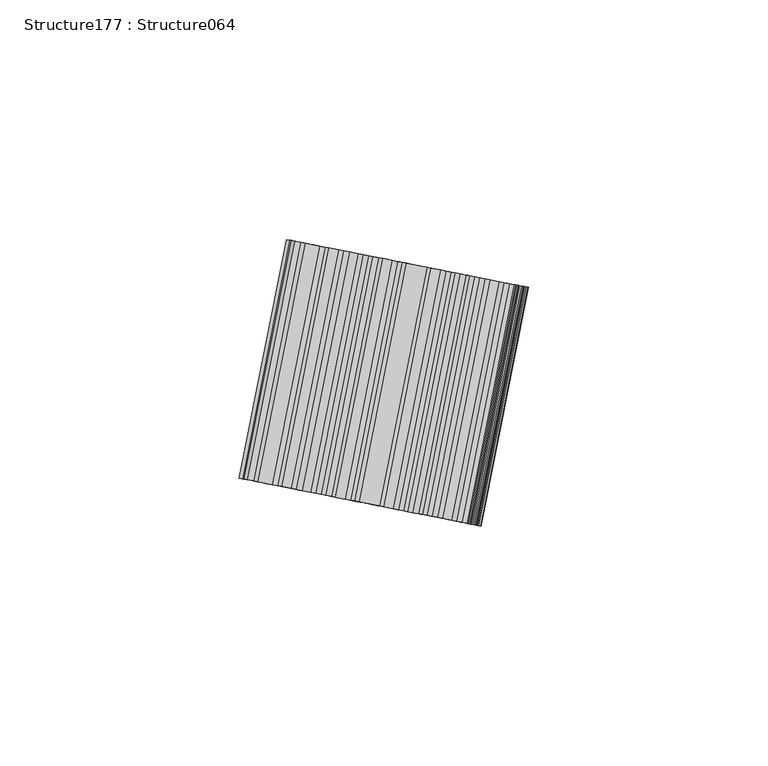
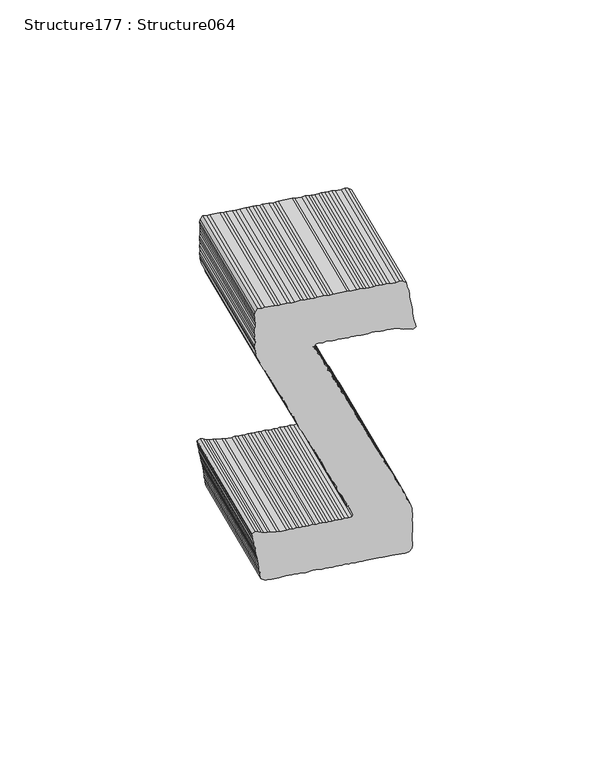
"""IFC4 building model written with IfcOpenShell, lengths in millimetres: proxy geometry, Structure177 : Structure064."""

from ifc_helpers import new_model, si_unit, frame, origin, place, context, project, spatial, polyline, outline, extrude, source, transform, mapped, element, save


def structure177_structure064_2659b349(model_context):
    return source(origin(), model_context, "Body", "SweptSolid", [
        extrude(outline(polyline([(1.0468911, 0.0), (1.5156229, -1.0820274), (1.8043049, -2.1128067), (2.0901183, -3.1435853), (2.6051551, -4.0455174), (2.8493861, -5.2553333), (3.1877265, -6.1090195), (3.6541636, -7.1898987), (3.9427132, -8.2211635), (4.2191677, -8.9614524), (4.5077172, -9.9927172), (4.9123563, -10.9617879), (5.4407688, -12.151916), (5.8915803, -12.9413769), (6.1839247, -13.9749819), (6.5222652, -14.8286681), (6.93803, -16.0827122), (6.1506863, -17.5841228), (5.2932054, -17.920123), (4.5699104, -18.4868046), (2.5398679, -19.6460344), (0.6051261, -20.450503), (-0.1861888, -20.9023732), (-1.1371166, -21.592076), (-2.1040693, -21.9975543), (-2.6501815, -22.6097456), (-3.6829912, -22.8991774), (-4.6802241, -23.7689754), (-6.728982, -24.6385514), (-8.4203751, -25.6043998), (-9.1948285, -26.3469824), (-10.1136222, -26.5713068), (-10.9983839, -27.3768795), (-12.0143321, -27.9570237), (-12.9842842, -28.3572492), (-14.6772223, -29.3239798), (-15.7544831, -29.7924481), (-16.4146115, -30.4697469), (-17.335259, -30.69513), (-18.3324919, -31.5649279), (-19.302135, -31.9649769), (-20.2522262, -32.6611676), (-21.2200154, -33.0601579), (-24.6065095, -34.993972), (-25.6665999, -35.7529763), (-26.4100648, -36.0238691), (-28.329799, -37.1201087), (-29.1634023, -37.7497805), (-31.7601264, -39.2326065), (-32.9547118, -39.7611059), (-34.3223762, -39.1993681), (-35.0653556, -38.4235023), (-35.5144028, -37.6371312), (-35.8683687, -36.4920268), (-36.4973321, -35.6510535), (-37.0123689, -34.7491213), (-37.5131478, -34.13693), (-39.0600226, -31.4280437), (-39.3479989, -30.3985003), (-40.2164293, -29.4029449), (-40.6060152, -28.7207023), (-41.0222655, -27.4665256), (-41.5390667, -26.5615036), (-41.9878049, -24.7280648), (-42.0390503, -23.8526173), (-42.0359182, -22.8104935), (-42.2127016, -21.7108988), (-42.4538005, -20.5058503), (-42.3247312, -19.6806799), (-42.5689621, -18.470864), (-42.7916546, -17.5556456), (-42.5507769, -16.6686772), (-42.8556578, -15.3447582), (-42.7933304, -13.3637113), (-43.1941746, -12.3969807), (-43.3090273, -10.3618179), (-43.1942185, -9.2555128), (-43.3048358, -8.2717882), (-43.3060717, -7.2256028), (-43.3026729, -6.1767708), (-43.7729495, -5.0956256), (-43.6411897, -4.2758844), (-43.7089007, -3.1140055), (-43.7694181, -1.9525258), (-43.9492913, 0.1921955), (-44.0598216, 1.1714625), (-44.1720707, 2.1587625), (-44.0444594, 2.9785932), (-44.3984253, 4.1236976), (-44.2202736, 5.1190765), (-44.2861307, 6.2820142), (-44.510455, 7.2008078), (-44.5086906, 8.244609), (-44.5569365, 9.1148038), (-44.7333239, 10.2101173), (-44.6853414, 11.4384714), (-44.8615522, 12.533476), (-44.9124887, 13.4091), (-45.202319, 14.4375847), (-45.1999797, 15.485402), (-45.2642049, 16.6447643), (-45.2012148, 18.6282384), (-45.470653, 19.3655683), (-45.4880877, 20.7048933), (-45.4254066, 21.6412998), (-45.6497309, 22.5600934), (-45.7639235, 23.5421861), (-45.7771226, 24.8769642), (-45.8922843, 25.8650592), (-46.0677895, 26.9588279), (-45.8232496, 27.8429708), (-46.1799517, 28.9885614), (-46.1609712, 30.7936608), (-46.2269608, 31.956113), (-46.5805309, 33.0969363), (-46.5805308, 34.1438275), (-46.404011, 35.1427817), (-46.8050316, 36.1098213), (-46.8077222, 37.1621416), (-46.6908831, 38.2691965), (-47.0972435, 39.237694), (-46.9643794, 40.0605242), (-47.1443851, 41.1578689), (-47.0937121, 42.3807938), (-47.2075517, 43.3622685), (-47.1442526, 44.2990279), (-47.139752, 45.3423429), (-48.2212036, 45.927387), (-49.2535279, 45.6378227), (-50.1403199, 44.8315002), (-51.1714083, 44.5426417), (-51.9611782, 44.0916537), (-52.7336452, 43.3506151), (-53.5249601, 42.8987448), (-54.6697556, 42.5449553), (-55.2837114, 42.0472663), (-56.1182853, 41.4178597), (-57.1339246, 40.8378919), (-58.0543958, 40.6121999), (-58.7808227, 40.0502857), (-59.9089331, 39.4060927), (-60.5188738, 38.90496), (-62.4382991, 37.8088968), (-63.5815496, 37.4559896), (-65.1620165, 36.5534842), (-65.9366463, 35.8112105), (-66.7264163, 35.3602224), (-67.982138, 34.94309), (-68.6436787, 34.2653943), (-70.2229097, 33.3635947), (-71.0918685, 32.2691634), (-71.7529686, 31.5892611), (-72.5914252, 30.9637834), (-73.3161772, 30.3946308), (-73.9653563, 29.4326676), (-75.1394627, 29.655447), (-75.5424242, 30.6258854), (-75.6545864, 31.6087278), (-75.9436214, 32.6401252), (-76.4771972, 33.831402), (-76.7505171, 34.5755297), (-77.391887, 35.6986962), (-77.7957308, 36.6706796), (-77.9533158, 37.4718819), (-78.7142155, 39.5872052), (-78.9373934, 40.5025561), (-79.5203607, 41.5234481), (-79.9227498, 42.4892965), (-80.2107262, 43.5188399), (-80.3734289, 44.3261341), (-80.7886205, 45.5784569), (-80.275479, 46.7786488), (-79.3887764, 47.5808228), (-78.3594525, 47.8727712), (-76.6646606, 48.8405604), (-75.8919741, 49.5776269), (-74.8114917, 50.0454765), (-73.9725488, 50.6736901), (-73.0703076, 51.1889034), (-72.3272387, 51.4640773), (-71.1375067, 51.9967708), (-70.2343386, 52.5125133), (-69.5077352, 53.0741186), (-68.6700282, 53.7016266), (-67.5898548, 54.1692996), (-65.7862995, 55.1991968), (-65.171681, 55.6993129), (-61.3380831, 57.8884398), (-60.482234, 58.2280154), (-59.6296065, 58.5682097), (-58.74105, 59.3714423), (-56.9374947, 60.4013394), (-56.1324952, 60.5651903), (-55.1302315, 61.4333539), (-54.3407706, 61.8841654), (-53.2624511, 62.3507799), (-52.4228902, 62.9793464), (-50.7144136, 63.6591163), (-49.5878481, 64.3024271), (-48.7478466, 64.9287869), (-46.9439823, 65.9588605), (-46.2038259, 66.2348296), (-45.3152694, 67.0380622), (-42.6079281, 68.5840548), (-41.6907663, 68.8119544), (-40.6881938, 69.6802944), (-39.4295156, 69.0489461), (-38.8664093, 68.3240193), (-38.3978541, 67.242301), (-37.9496891, 66.4574748), (-37.5491539, 65.4905678), (-36.9661866, 64.4696758), (-36.2903432, 63.8128137), (-35.7761886, 62.9124265), (-35.3048103, 61.8257644), (-34.6803018, 60.9933102), (-34.0695237, 59.3970413), (-33.261701, 58.5090572), (-32.7927929, 57.4267209), (-32.5233547, 56.689391), (-31.8933326, 54.7996727), (-31.7828479, 52.7685714), (-31.3793545, 51.8058121), (-31.3631118, 50.4649869), (-31.3171157, 49.5980145), (-31.4264549, 48.4821308), (-31.3141162, 47.4989794), (-31.3141162, 46.4520882), (-31.0267579, 45.422192), (-31.2049097, 44.4268131), (-30.8021246, 43.4566836), (-30.7842044, 42.1172261), (-30.6228702, 41.3087407), (-30.5595711, 40.1517177), (-30.5105755, 39.2794926), (-30.3833162, 38.0090276), (-30.6263112, 37.1257669), (-30.2862073, 36.2661222), (-30.1608458, 34.995393), (-30.3373657, 33.9964388), (-30.2234822, 33.0141696), (-30.0459931, 31.9133391), (-29.9811052, 30.7564039), (-29.5819384, 28.7414145), (-29.9381551, 27.7930904), (-29.6441333, 26.760853), (-29.5336486, 25.776643), (-29.5176693, 24.4405843), (-29.3570847, 23.6341293), (-29.1790199, 22.5401834), (-29.2917131, 21.4244331), (-29.1327604, 20.6215534), (-29.1349233, 19.5734271), (-29.1347469, 18.526227), (-28.9548737, 17.4283968), (-29.0688898, 16.3163981), (-28.7320943, 15.4618297), (-28.8282773, 14.0617223), (-28.6024079, 13.1438109), (-28.602012, 12.0926387), (-28.5377868, 10.9332764), (-28.4256246, 9.950434), (-28.4919233, 9.0189274), (-28.2493698, 7.8077438), (-28.2512237, 6.759794), (-28.0397896, 5.0821725), (-27.8495403, 3.7013993), (-27.9605569, 2.5841479), (-27.8483946, 0.5544144), (-27.5760439, -0.1837108), (-27.7373342, -1.4698022), (-27.5098777, -2.3933632), (-27.6243354, -3.5060236), (-27.2216373, -4.4716955), (-27.1105346, -5.4555526), (-27.2876724, -7.5017509), (-27.0481186, -8.7076817), (-26.9810702, -9.8719878), (-26.9826152, -10.9197612), (-26.6425534, -11.7728741), (-26.807419, -13.0605974), (-26.5826093, -15.0264147), (-26.4179657, -15.8371077), (-25.8082015, -16.3825573), (-24.7266595, -15.9136931), (-23.775069, -15.221563), (-22.9231042, -14.8837959), (-22.020863, -14.3685827), (-21.0674186, -13.675394), (-20.1480518, -13.4527911), (-19.3104319, -12.8208257), (-18.5688209, -12.5509915), (-17.6208926, -11.856036), (-16.8936265, -11.2920035), (-15.6368462, -10.876725), (-15.0882173, -10.2610477), (-14.0100742, -9.7941244), (-13.1062881, -9.278029), (-12.2668598, -8.6499477), (-11.2365667, -8.3640018), (-10.625434, -7.861369), (-9.4293036, -7.3319873), (-8.7697485, -6.6529671), (-7.7363655, -6.3652568), (-5.9325012, -5.3351832), (-5.1589301, -4.5910555), (-3.5987234, -3.3997786), (-2.9839284, -2.8999714), (-1.9218077, -2.1402175), (-1.3699598, -1.533765), (-0.8395609, -0.6285667), (0.0, 0.0), (1.0468911, 0.0)])), frame((-1782.3886746, 234822.2083705, 404.8484925), z_axis=(0.19466222296394123, 0.9808703374813295, 0.0), x_axis=(-0.8517775151981756, 0.16904263310167944, -0.49588270064287676)), (0.0, 0.0, 1.0), 50.8),
    ])


if __name__ == "__main__":
    model = new_model("IFC4")
    model_context = context("Model", 3, world=origin())
    ifc_project = project(units=[si_unit("LENGTHUNIT", "METRE", prefix="MILLI")], contexts=[model_context])
    site = spatial("IfcSite", under=ifc_project)
    building = spatial("IfcBuilding", under=site)
    placement = place(None, origin())
    structure177_structure064_shape = structure177_structure064_2659b349(model_context)
    element("IfcBuildingElementProxy", 1, Name="Structure177 : Structure064", ObjectType="Structure177 : Structure064", at=placement, inside=building, context=model_context, shape_type="MappedRepresentation", body=[
        mapped(structure177_structure064_shape, transform((0.0, 0.0, 0.0), x_axis=(1.0, 0.0, 0.0), y_axis=(0.0, 1.0, 0.0), z_axis=(0.0, 0.0, 1.0))),
    ])
    save(model, "model.ifc")

# Revit data of these elements
# Type "Structure177 : Structure064"
#   NameOverride = "Structure064"
# Element 1 (IfcBuildingElementProxy, "Structure177 : Structure064")
#   Materials on its faces: "BRUSHED ALUMINUM LETTERING"
# Materials
#   "BRUSHED ALUMINUM LETTERING": class "Unassigned", colour RGB 169 181 186, transparency 0, Cost = 0
